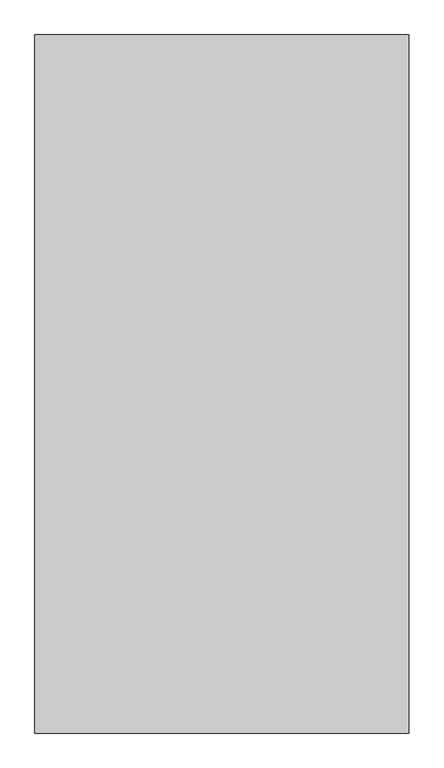
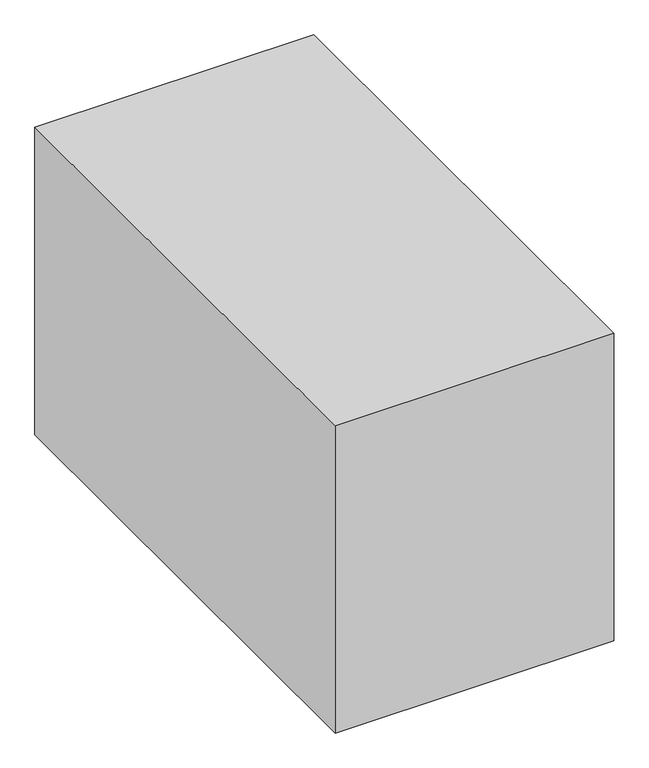
"""IFC4 building model written with IfcOpenShell, lengths in millimetres: proxy geometry, Space Planning Box_hec : Space Planning Box_hec."""

import ifcopenshell
import ifcopenshell.guid

model = None  # the IFC model being written
_history = None  # IfcOwnerHistory: only IFC2X3 demands one
_inside = {}  # id of a spatial element -> (the spatial element, [elements in it])
_under = {}  # id of a project, library or spatial element -> (it, [spatial elements below it])
_declared = {}  # id of a project -> (the project, [libraries it declares])
_typed = {}  # id of a type object -> (the type object, [elements of that type])
_made_of = {}  # id of a material, layer set ... -> (it, [elements and type objects made of it])


def new_model(schema):
    """Start an empty IFC model of exactly this schema.

    Asked for "IFC4X3", IfcOpenShell would pick the latest addendum, in which some entities
    have other attributes; the version numbers below select the first issue.
    IFC2X3 requires an IfcOwnerHistory on every rooted entity: one is made here for all.
    """
    global model, _history
    if schema == "IFC4X3":
        model = ifcopenshell.file(schema_version=(4, 3, 0, 0))
    else:
        model = ifcopenshell.file(schema=schema)
    _inside.clear()
    _under.clear()
    _declared.clear()
    _typed.clear()
    _made_of.clear()
    _history = None
    if model.schema == "IFC2X3":
        org = make("IfcOrganization", Name="unknown")
        user = make(
            "IfcPersonAndOrganization",
            ThePerson=make("IfcPerson", FamilyName="unknown"),
            TheOrganization=org,
        )
        app = make(
            "IfcApplication",
            ApplicationDeveloper=org,
            Version="unknown",
            ApplicationFullName="unknown",
            ApplicationIdentifier="unknown",
        )
        _history = make(
            "IfcOwnerHistory",
            OwningUser=user,
            OwningApplication=app,
            ChangeAction="ADDED",
            CreationDate=0,
        )
    return model


def make(cls, **values):
    """One entity of the class cls with the attributes given. An attribute that is None is left unset."""
    return model.create_entity(
        cls, **{name: value for name, value in values.items() if value is not None}
    )


def rooted(cls, **values):
    """An entity with a GlobalId (a new one), such as an element, a storey or a relation."""
    return make(cls, GlobalId=ifcopenshell.guid.new(), OwnerHistory=_history, **values)


def si_unit(unit_type, name, prefix=None):
    """IfcSIUnit, for example si_unit("LENGTHUNIT", "METRE", prefix="MILLI")."""
    return make("IfcSIUnit", UnitType=unit_type, Prefix=prefix, Name=name)


def assignment(units):
    """IfcUnitAssignment: the units of a project."""
    return None if units is None else make("IfcUnitAssignment", Units=units)


def point(xyz):
    """IfcCartesianPoint."""
    return None if xyz is None else make("IfcCartesianPoint", Coordinates=xyz)


def direction(xyz):
    """IfcDirection."""
    return None if xyz is None else make("IfcDirection", DirectionRatios=xyz)


def frame(location, z_axis=None, x_axis=None):
    """IfcAxis2Placement3D, a coordinate frame: its origin and axes. An axis left out is left unset."""
    return make(
        "IfcAxis2Placement3D",
        Location=point(location),
        Axis=direction(z_axis),
        RefDirection=direction(x_axis),
    )


def origin():
    """The frame at (0, 0, 0) with its axes left unset."""
    return frame((0.0, 0.0, 0.0))


def origin_with_axes():
    """The frame at (0, 0, 0) with the z axis (0, 0, 1) and the x axis (1, 0, 0) written out."""
    return frame((0.0, 0.0, 0.0), z_axis=(0.0, 0.0, 1.0), x_axis=(1.0, 0.0, 0.0))


def place(relative_to, where):
    """IfcLocalPlacement: puts the frame where relative to a parent placement (None: the world)."""
    return make(
        "IfcLocalPlacement", PlacementRelTo=relative_to, RelativePlacement=where
    )


def context(
    kind, dimensions, precision=None, world=None, true_north=None, identifier=None
):
    """IfcGeometricRepresentationContext, for example the 3D "Model" context."""
    return make(
        "IfcGeometricRepresentationContext",
        ContextIdentifier=identifier,
        ContextType=kind,
        CoordinateSpaceDimension=dimensions,
        Precision=precision,
        WorldCoordinateSystem=world,
        TrueNorth=true_north,
    )


def project(units=None, contexts=None):
    """IfcProject with its units and contexts."""
    return rooted(
        "IfcProject",
        Name="project",
        RepresentationContexts=contexts,
        UnitsInContext=assignment(units),
    )


def spatial(cls, under=None, at=None, **own):
    """A site, building, storey or space (cls), placed at a placement, below another one or the project."""
    s = rooted(cls, ObjectPlacement=at, **own)
    if under is not None:
        _under.setdefault(under.id(), (under, []))[1].append(s)
    return s


def polyline(points):
    """IfcPolyline through the points."""
    return make("IfcPolyline", Points=[point(p) for p in points])


def outline(outer, holes=None, kind="AREA"):
    """IfcArbitraryClosedProfileDef: a profile drawn as a closed curve; with holes, ...WithVoids."""
    if holes is None:
        return make("IfcArbitraryClosedProfileDef", ProfileType=kind, OuterCurve=outer)
    return make(
        "IfcArbitraryProfileDefWithVoids",
        ProfileType=kind,
        OuterCurve=outer,
        InnerCurves=holes,
    )


def extrude(swept, where, along, depth):
    """IfcExtrudedAreaSolid: the profile swept, set in the frame where, extruded along a direction by depth."""
    return make(
        "IfcExtrudedAreaSolid",
        SweptArea=swept,
        Position=where,
        ExtrudedDirection=direction(along),
        Depth=depth,
    )


def shape(context_of_items, identifier, shape_type, items):
    """IfcShapeRepresentation: the items that make up one representation, for example the "Body"."""
    return make(
        "IfcShapeRepresentation",
        ContextOfItems=context_of_items,
        RepresentationIdentifier=identifier,
        RepresentationType=shape_type,
        Items=items,
    )


def source(mapping_origin, context_of_items, identifier, shape_type, items):
    """IfcRepresentationMap: a shape defined once, which mapped items show again and again."""
    return make(
        "IfcRepresentationMap",
        MappingOrigin=mapping_origin,
        MappedRepresentation=shape(context_of_items, identifier, shape_type, items),
    )


def transform(
    local_origin,
    x_axis=None,
    y_axis=None,
    z_axis=None,
    scale=None,
    scale2=None,
    scale3=None,
    uniform=True,
):
    """IfcCartesianTransformationOperator3D, or its non-uniform kind. x_axis, y_axis, z_axis: its Axis1, 2, 3."""
    if uniform:
        return make(
            "IfcCartesianTransformationOperator3D",
            Axis1=direction(x_axis),
            Axis2=direction(y_axis),
            LocalOrigin=point(local_origin),
            Scale=scale,
            Axis3=direction(z_axis),
        )
    return make(
        "IfcCartesianTransformationOperator3DnonUniform",
        Axis1=direction(x_axis),
        Axis2=direction(y_axis),
        LocalOrigin=point(local_origin),
        Scale=scale,
        Axis3=direction(z_axis),
        Scale2=scale2,
        Scale3=scale3,
    )


def mapped(mapping_source, mapping_target):
    """IfcMappedItem: shows the shape of a source again, moved by a transform."""
    return make(
        "IfcMappedItem", MappingSource=mapping_source, MappingTarget=mapping_target
    )


def made_of(thing, what):
    """Note that an element or type object is made of a material, layer set ...; save() writes the relation."""
    if what is not None:
        _made_of.setdefault(what.id(), (what, []))[1].append(thing)
    return thing


def element(
    cls,
    number,
    at=None,
    inside=None,
    cuts=None,
    type_object=None,
    material=None,
    context=None,
    identifier="Body",
    shape_type=None,
    held_by="IfcProductDefinitionShape",
    body=None,
    shapes=None,
    **own,
):
    """One element of the class cls, such as IfcWall. Its Tag is "e" and its number.

    at: its placement. inside: the storey or other place that contains it. cuts: it is an
    opening in that element (IfcRelVoidsElement). A single representation is given by context,
    identifier, shape_type and body (its items); several are given by shapes. held_by: the class
    of the entity that holds the representations. save() writes the other relations.
    """
    e = rooted(cls, Tag="e%d" % number, ObjectPlacement=at, **own)
    if body is not None:
        shapes = [shape(context, identifier, shape_type, body)]
    if shapes is not None:
        e.Representation = make(held_by, Representations=shapes)
    if inside is not None:
        _inside.setdefault(inside.id(), (inside, []))[1].append(e)
    if cuts is not None:
        rooted(
            "IfcRelVoidsElement", RelatingBuildingElement=cuts, RelatedOpeningElement=e
        )
    if type_object is not None:
        _typed.setdefault(type_object.id(), (type_object, []))[1].append(e)
    return made_of(e, material)


def aggregate(whole, parts):
    """IfcRelAggregates: a whole, such as a stair, and the parts it consists of."""
    return rooted("IfcRelAggregates", RelatingObject=whole, RelatedObjects=parts)


def save(model, path):
    """Write the relations noted so far, then the file.

    IfcRelAggregates (storeys below a building ...), IfcRelContainedInSpatialStructure (elements
    in a storey), IfcRelDefinesByType, IfcRelAssociatesMaterial and IfcRelDeclares: one each for
    every whole, place, type object, material and project.
    """
    for whole, parts in _under.values():
        aggregate(whole, parts)
    for where, things in _inside.values():
        rooted(
            "IfcRelContainedInSpatialStructure",
            RelatedElements=things,
            RelatingStructure=where,
        )
    for kind, things in _typed.values():
        rooted("IfcRelDefinesByType", RelatedObjects=things, RelatingType=kind)
    for what, things in _made_of.values():
        rooted("IfcRelAssociatesMaterial", RelatedObjects=things, RelatingMaterial=what)
    for by, libraries in _declared.values():
        rooted("IfcRelDeclares", RelatingContext=by, RelatedDefinitions=libraries)
    model.write(path)


def generic_models_f42d0df8(model_context):
    return source(origin(), model_context, "Body", "SweptSolid", [
        extrude(outline(polyline([(1500.0, 2800.0), (1500.0, -2800.0), (-1500.0, -2800.0), (-1500.0, 2800.0), (1500.0, 2800.0)])), origin_with_axes(), (0.0, 0.0, 1.0), 3500.0),
    ])


if __name__ == "__main__":
    model = new_model("IFC4")
    model_context = context("Model", 3, world=origin())
    ifc_project = project(units=[si_unit("LENGTHUNIT", "METRE", prefix="MILLI")], contexts=[model_context])
    site = spatial("IfcSite", under=ifc_project)
    building = spatial("IfcBuilding", under=site)
    placement = place(None, origin())
    generic_models_shape = generic_models_f42d0df8(model_context)
    element("IfcBuildingElementProxy", 1, Name="Space Planning Box_hec : Space Planning Box_hec", ObjectType="Space Planning Box_hec : Space Planning Box_hec", at=placement, inside=building, context=model_context, shape_type="MappedRepresentation", body=[
        mapped(generic_models_shape, transform((0.0, 0.0, 0.0), x_axis=(1.0, 0.0, 0.0), y_axis=(0.0, 1.0, 0.0), z_axis=(0.0, 0.0, 1.0))),
    ])
    save(model, "model.ifc")

# Revit data of these elements
# Type "Space Planning Box_hec : Space Planning Box_hec"
#   Type Comments = "..."
#   Room Name [instance default] = "?"
#   Interior Finish [instance default] = ""
#   Exterior Finish [instance default] = ""
#   Department [instance default] = ""
#   Assembly Code = "..."
#   ceiling height [instance default] = 0
#   Width [instance default] = 1524 mm
#   Program Area [instance default] = 0.00 m²
#   Length [instance default] = 1524 mm
#   Height [instance default] = 1524 mm
#   Area [instance default] = 2.32258 m²
#   Fill Color [instance default] = Cyan
#   Default Elevation = 0
# Element 1 (IfcBuildingElementProxy, "Space Planning Box_hec : Space Planning Box_hec")
#   Room Name = "Toilet(F)"
#   Exterior Finish = "RF1..N/A,,N/A..N/A..N/A"
#   Department = "AR"
#   Width = 3000 mm
#   Program Area = 16.80 m²
#   Length = 5600 mm
#   Height = 3500 mm
#   Area = 16.80 m²
#   Materials on its faces: "Cyan"
# Materials
#   "Cyan": class "Generic", colour RGB 0 255 255, transparency 0.2, Cost = 0
